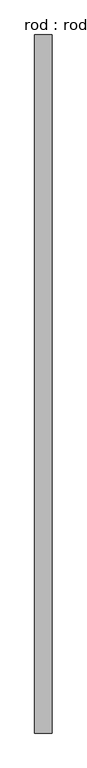
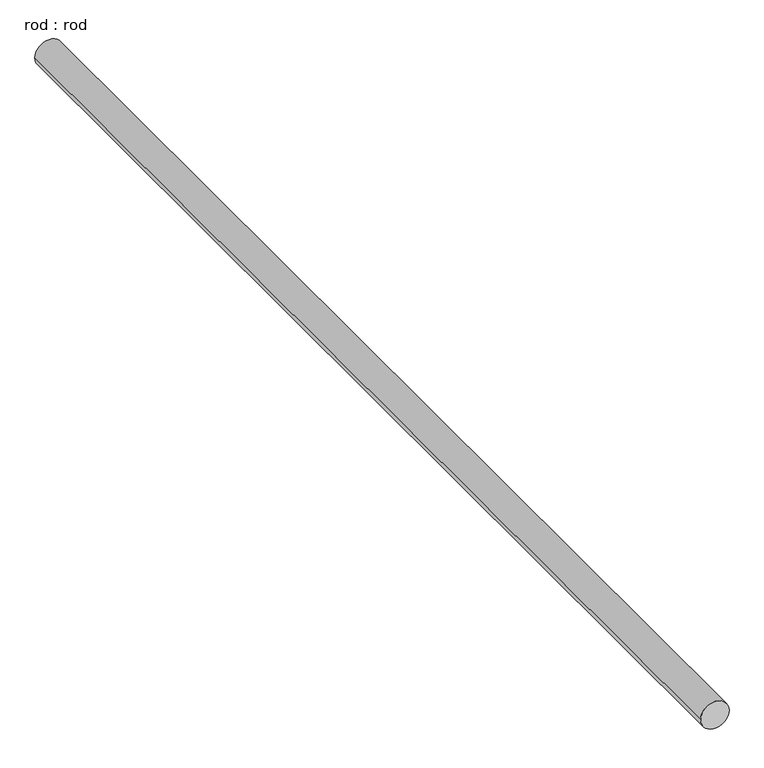
"""IFC4 building model written with IfcOpenShell, lengths in millimetres: proxy geometry, rod : rod."""

import ifcopenshell
import ifcopenshell.guid

model = None  # the IFC model being written
_history = None  # IfcOwnerHistory: only IFC2X3 demands one
_inside = {}  # id of a spatial element -> (the spatial element, [elements in it])
_under = {}  # id of a project, library or spatial element -> (it, [spatial elements below it])
_declared = {}  # id of a project -> (the project, [libraries it declares])
_typed = {}  # id of a type object -> (the type object, [elements of that type])
_made_of = {}  # id of a material, layer set ... -> (it, [elements and type objects made of it])


def new_model(schema):
    """Start an empty IFC model of exactly this schema.

    Asked for "IFC4X3", IfcOpenShell would pick the latest addendum, in which some entities
    have other attributes; the version numbers below select the first issue.
    IFC2X3 requires an IfcOwnerHistory on every rooted entity: one is made here for all.
    """
    global model, _history
    if schema == "IFC4X3":
        model = ifcopenshell.file(schema_version=(4, 3, 0, 0))
    else:
        model = ifcopenshell.file(schema=schema)
    _inside.clear()
    _under.clear()
    _declared.clear()
    _typed.clear()
    _made_of.clear()
    _history = None
    if model.schema == "IFC2X3":
        org = make("IfcOrganization", Name="unknown")
        user = make(
            "IfcPersonAndOrganization",
            ThePerson=make("IfcPerson", FamilyName="unknown"),
            TheOrganization=org,
        )
        app = make(
            "IfcApplication",
            ApplicationDeveloper=org,
            Version="unknown",
            ApplicationFullName="unknown",
            ApplicationIdentifier="unknown",
        )
        _history = make(
            "IfcOwnerHistory",
            OwningUser=user,
            OwningApplication=app,
            ChangeAction="ADDED",
            CreationDate=0,
        )
    return model


def make(cls, **values):
    """One entity of the class cls with the attributes given. An attribute that is None is left unset."""
    return model.create_entity(
        cls, **{name: value for name, value in values.items() if value is not None}
    )


def rooted(cls, **values):
    """An entity with a GlobalId (a new one), such as an element, a storey or a relation."""
    return make(cls, GlobalId=ifcopenshell.guid.new(), OwnerHistory=_history, **values)


def si_unit(unit_type, name, prefix=None):
    """IfcSIUnit, for example si_unit("LENGTHUNIT", "METRE", prefix="MILLI")."""
    return make("IfcSIUnit", UnitType=unit_type, Prefix=prefix, Name=name)


def assignment(units):
    """IfcUnitAssignment: the units of a project."""
    return None if units is None else make("IfcUnitAssignment", Units=units)


def point(xyz):
    """IfcCartesianPoint."""
    return None if xyz is None else make("IfcCartesianPoint", Coordinates=xyz)


def direction(xyz):
    """IfcDirection."""
    return None if xyz is None else make("IfcDirection", DirectionRatios=xyz)


def frame(location, z_axis=None, x_axis=None):
    """IfcAxis2Placement3D, a coordinate frame: its origin and axes. An axis left out is left unset."""
    return make(
        "IfcAxis2Placement3D",
        Location=point(location),
        Axis=direction(z_axis),
        RefDirection=direction(x_axis),
    )


def frame_2d(location, x_axis=None):
    """IfcAxis2Placement2D, a coordinate frame in the plane: its origin and x axis."""
    return make(
        "IfcAxis2Placement2D", Location=point(location), RefDirection=direction(x_axis)
    )


def origin():
    """The frame at (0, 0, 0) with its axes left unset."""
    return frame((0.0, 0.0, 0.0))


def place(relative_to, where):
    """IfcLocalPlacement: puts the frame where relative to a parent placement (None: the world)."""
    return make(
        "IfcLocalPlacement", PlacementRelTo=relative_to, RelativePlacement=where
    )


def context(
    kind, dimensions, precision=None, world=None, true_north=None, identifier=None
):
    """IfcGeometricRepresentationContext, for example the 3D "Model" context."""
    return make(
        "IfcGeometricRepresentationContext",
        ContextIdentifier=identifier,
        ContextType=kind,
        CoordinateSpaceDimension=dimensions,
        Precision=precision,
        WorldCoordinateSystem=world,
        TrueNorth=true_north,
    )


def project(units=None, contexts=None):
    """IfcProject with its units and contexts."""
    return rooted(
        "IfcProject",
        Name="project",
        RepresentationContexts=contexts,
        UnitsInContext=assignment(units),
    )


def spatial(cls, under=None, at=None, **own):
    """A site, building, storey or space (cls), placed at a placement, below another one or the project."""
    s = rooted(cls, ObjectPlacement=at, **own)
    if under is not None:
        _under.setdefault(under.id(), (under, []))[1].append(s)
    return s


def circle_curve(where, radius):
    """IfcCircle in the frame where."""
    return make("IfcCircle", Position=where, Radius=radius)


def trimmed(basis, trim1, trim2, sense, master):
    """IfcTrimmedCurve: the piece of a basis curve between two trims."""
    return make(
        "IfcTrimmedCurve",
        BasisCurve=basis,
        Trim1=trim1,
        Trim2=trim2,
        SenseAgreement=sense,
        MasterRepresentation=master,
    )


def segment(curve, same_sense, transition):
    """IfcCompositeCurveSegment."""
    return make(
        "IfcCompositeCurveSegment",
        Transition=transition,
        SameSense=same_sense,
        ParentCurve=curve,
    )


def composite_curve(segments, self_intersect=None):
    """IfcCompositeCurve: segments joined end to end."""
    return make("IfcCompositeCurve", Segments=segments, SelfIntersect=self_intersect)


def outline(outer, holes=None, kind="AREA"):
    """IfcArbitraryClosedProfileDef: a profile drawn as a closed curve; with holes, ...WithVoids."""
    if holes is None:
        return make("IfcArbitraryClosedProfileDef", ProfileType=kind, OuterCurve=outer)
    return make(
        "IfcArbitraryProfileDefWithVoids",
        ProfileType=kind,
        OuterCurve=outer,
        InnerCurves=holes,
    )


def extrude(swept, where, along, depth):
    """IfcExtrudedAreaSolid: the profile swept, set in the frame where, extruded along a direction by depth."""
    return make(
        "IfcExtrudedAreaSolid",
        SweptArea=swept,
        Position=where,
        ExtrudedDirection=direction(along),
        Depth=depth,
    )


def shape(context_of_items, identifier, shape_type, items):
    """IfcShapeRepresentation: the items that make up one representation, for example the "Body"."""
    return make(
        "IfcShapeRepresentation",
        ContextOfItems=context_of_items,
        RepresentationIdentifier=identifier,
        RepresentationType=shape_type,
        Items=items,
    )


def source(mapping_origin, context_of_items, identifier, shape_type, items):
    """IfcRepresentationMap: a shape defined once, which mapped items show again and again."""
    return make(
        "IfcRepresentationMap",
        MappingOrigin=mapping_origin,
        MappedRepresentation=shape(context_of_items, identifier, shape_type, items),
    )


def transform(
    local_origin,
    x_axis=None,
    y_axis=None,
    z_axis=None,
    scale=None,
    scale2=None,
    scale3=None,
    uniform=True,
):
    """IfcCartesianTransformationOperator3D, or its non-uniform kind. x_axis, y_axis, z_axis: its Axis1, 2, 3."""
    if uniform:
        return make(
            "IfcCartesianTransformationOperator3D",
            Axis1=direction(x_axis),
            Axis2=direction(y_axis),
            LocalOrigin=point(local_origin),
            Scale=scale,
            Axis3=direction(z_axis),
        )
    return make(
        "IfcCartesianTransformationOperator3DnonUniform",
        Axis1=direction(x_axis),
        Axis2=direction(y_axis),
        LocalOrigin=point(local_origin),
        Scale=scale,
        Axis3=direction(z_axis),
        Scale2=scale2,
        Scale3=scale3,
    )


def mapped(mapping_source, mapping_target):
    """IfcMappedItem: shows the shape of a source again, moved by a transform."""
    return make(
        "IfcMappedItem", MappingSource=mapping_source, MappingTarget=mapping_target
    )


def made_of(thing, what):
    """Note that an element or type object is made of a material, layer set ...; save() writes the relation."""
    if what is not None:
        _made_of.setdefault(what.id(), (what, []))[1].append(thing)
    return thing


def element(
    cls,
    number,
    at=None,
    inside=None,
    cuts=None,
    type_object=None,
    material=None,
    context=None,
    identifier="Body",
    shape_type=None,
    held_by="IfcProductDefinitionShape",
    body=None,
    shapes=None,
    **own,
):
    """One element of the class cls, such as IfcWall. Its Tag is "e" and its number.

    at: its placement. inside: the storey or other place that contains it. cuts: it is an
    opening in that element (IfcRelVoidsElement). A single representation is given by context,
    identifier, shape_type and body (its items); several are given by shapes. held_by: the class
    of the entity that holds the representations. save() writes the other relations.
    """
    e = rooted(cls, Tag="e%d" % number, ObjectPlacement=at, **own)
    if body is not None:
        shapes = [shape(context, identifier, shape_type, body)]
    if shapes is not None:
        e.Representation = make(held_by, Representations=shapes)
    if inside is not None:
        _inside.setdefault(inside.id(), (inside, []))[1].append(e)
    if cuts is not None:
        rooted(
            "IfcRelVoidsElement", RelatingBuildingElement=cuts, RelatedOpeningElement=e
        )
    if type_object is not None:
        _typed.setdefault(type_object.id(), (type_object, []))[1].append(e)
    return made_of(e, material)


def aggregate(whole, parts):
    """IfcRelAggregates: a whole, such as a stair, and the parts it consists of."""
    return rooted("IfcRelAggregates", RelatingObject=whole, RelatedObjects=parts)


def save(model, path):
    """Write the relations noted so far, then the file.

    IfcRelAggregates (storeys below a building ...), IfcRelContainedInSpatialStructure (elements
    in a storey), IfcRelDefinesByType, IfcRelAssociatesMaterial and IfcRelDeclares: one each for
    every whole, place, type object, material and project.
    """
    for whole, parts in _under.values():
        aggregate(whole, parts)
    for where, things in _inside.values():
        rooted(
            "IfcRelContainedInSpatialStructure",
            RelatedElements=things,
            RelatingStructure=where,
        )
    for kind, things in _typed.values():
        rooted("IfcRelDefinesByType", RelatedObjects=things, RelatingType=kind)
    for what, things in _made_of.values():
        rooted("IfcRelAssociatesMaterial", RelatedObjects=things, RelatingMaterial=what)
    for by, libraries in _declared.values():
        rooted("IfcRelDeclares", RelatingContext=by, RelatedDefinitions=libraries)
    model.write(path)


def rod_rod_c51c1d5e(model_context):
    return source(origin(), model_context, "Body", "SweptSolid", [
        extrude(outline(composite_curve([segment(trimmed(circle_curve(frame_2d((0.0108462, 0.0)), 200.0), [point((0.0108462, 200.0))], [point((0.0108462, -200.0))], False, "CARTESIAN"), True, "CONTINUOUS"), segment(trimmed(circle_curve(frame_2d((0.0108462, 0.0)), 200.0), [point((0.0108462, -200.0))], [point((0.0108462, 200.0))], False, "CARTESIAN"), True, "CONTINUOUS")], self_intersect=False)), frame((0.0, -4010.2880314, 0.0), z_axis=(0.0, 1.0, 0.0), x_axis=(0.0, 0.0, 1.0)), (0.0, 0.0, 1.0), 16206.0332935),
    ])


if __name__ == "__main__":
    model = new_model("IFC4")
    model_context = context("Model", 3, world=origin())
    ifc_project = project(units=[si_unit("LENGTHUNIT", "METRE", prefix="MILLI")], contexts=[model_context])
    site = spatial("IfcSite", under=ifc_project)
    building = spatial("IfcBuilding", under=site)
    placement = place(None, origin())
    rod_rod_shape = rod_rod_c51c1d5e(model_context)
    element("IfcBuildingElementProxy", 1, Name="rod : rod", ObjectType="rod : rod", at=placement, inside=building, context=model_context, shape_type="MappedRepresentation", body=[
        mapped(rod_rod_shape, transform((0.0, 0.0, 0.0), x_axis=(1.0, 0.0, 0.0), y_axis=(0.0, 1.0, 0.0), z_axis=(0.0, 0.0, 1.0))),
    ])
    save(model, "model.ifc")

# Revit data of these elements
# Type "rod : rod"
#   Default Elevation = 0
